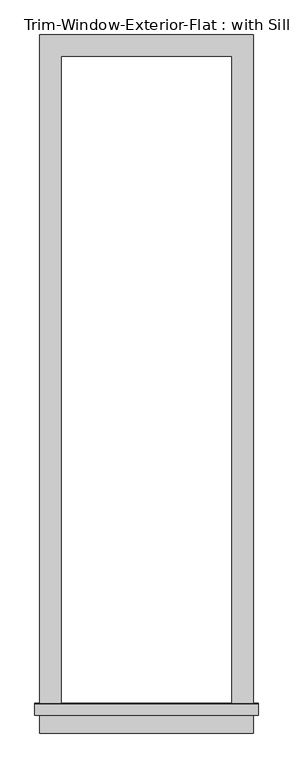
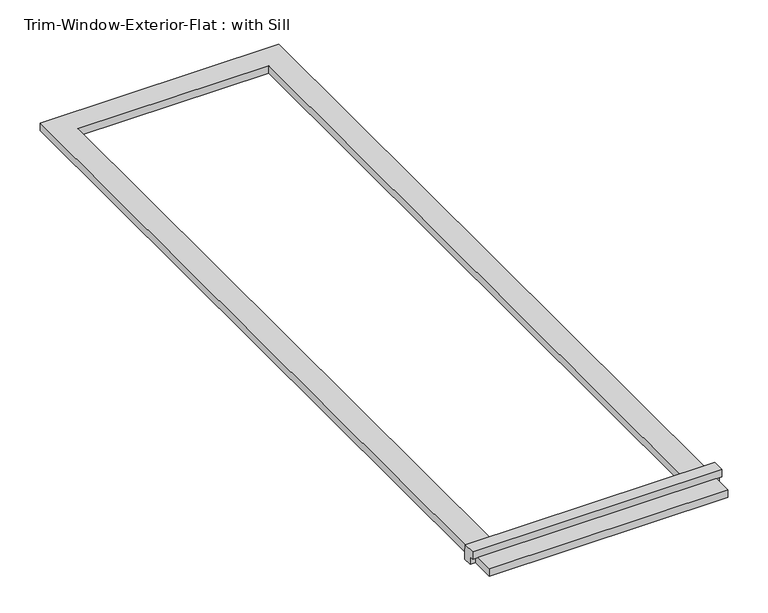
"""IFC4 building model written with IfcOpenShell, lengths in millimetres: proxy geometry, Trim-Window-Exterior-Flat : with Sill."""

from ifc_helpers import new_model, si_unit, frame, origin, origin_with_axes, place, context, project, spatial, polyline, outline, extrude, source, transform, mapped, element, save


def trim_window_exterior_flat_with_sill_cd637d81(model_context):
    return source(origin(), model_context, "Body", "SweptSolid", [
        extrude(outline(polyline([(285.75, -1749.3823709), (285.75, -1806.5323709), (-285.75, -1806.5323709), (-285.75, -1749.3823709), (285.75, -1749.3823709)])), origin_with_axes(), (0.0, 0.0, 1.0), 19.05),
        extrude(outline(polyline([(-1758.95, 38.1), (-1729.6580645, 38.1), (-1727.2, 19.05), (-1727.2, 0.0), (-1749.3823709, 0.0), (-1749.3823709, 19.05), (-1758.95, 19.05), (-1758.95, 38.1)])), frame((-298.45, 0.0, 0.0), z_axis=(1.0, 0.0, 0.0), x_axis=(0.0, 1.0, 0.0)), (0.0, 0.0, 1.0), 596.9),
        extrude(outline(polyline([(-285.75, 57.15), (285.75, 57.15), (285.75, -1727.2), (228.6, -1727.2), (228.6, 0.0), (-228.6, 0.0), (-228.6, -1727.2), (-285.75, -1727.2), (-285.75, 57.15)])), origin_with_axes(), (0.0, 0.0, 1.0), 19.05),
    ])


if __name__ == "__main__":
    model = new_model("IFC4")
    model_context = context("Model", 3, world=origin())
    ifc_project = project(units=[si_unit("LENGTHUNIT", "METRE", prefix="MILLI")], contexts=[model_context])
    site = spatial("IfcSite", under=ifc_project)
    building = spatial("IfcBuilding", under=site)
    placement = place(None, origin())
    trim_window_exterior_flat_with_sill_shape = trim_window_exterior_flat_with_sill_cd637d81(model_context)
    element("IfcBuildingElementProxy", 1, Name="Trim-Window-Exterior-Flat : with Sill", ObjectType="Trim-Window-Exterior-Flat : with Sill", at=placement, inside=building, context=model_context, shape_type="MappedRepresentation", body=[
        mapped(trim_window_exterior_flat_with_sill_shape, transform((0.0, 0.0, 0.0), x_axis=(1.0, 0.0, 0.0), y_axis=(0.0, 1.0, 0.0), z_axis=(0.0, 0.0, 1.0))),
    ])
    save(model, "model.ifc")

# Revit data of these elements
# Type "Trim-Window-Exterior-Flat : with Sill"
#   Trim Width = 0' - 2 1/4"
#   Trim Thickness_Picture Frame = 0' - 1 1/4"
#   Trim Thickness_with Sill = 0' - 0 3/4"
#   Sill Thickness = 0' - 1 1/4"
#   Opening Width [instance default] = 2' - 0"
#   Opening Height [instance default] = 3' - 0"
#   Default Elevation = 4' - 0"
#   Sill = yes
#   Picture Frame = no
#   Trim Material [instance default] = none
# Element 1 (IfcBuildingElementProxy, "Trim-Window-Exterior-Flat : with Sill")
#   Opening Width = 1' - 6"
#   Opening Height = 5' - 8"
#   Trim Material = 1X WOOD COMPOSITE TRIM
#   Materials on its faces: "1X WOOD COMPOSITE TRIM"
# Materials
#   "1X WOOD COMPOSITE TRIM": class "Generic", colour RGB 88 61 61, transparency 0, Cost = 0
